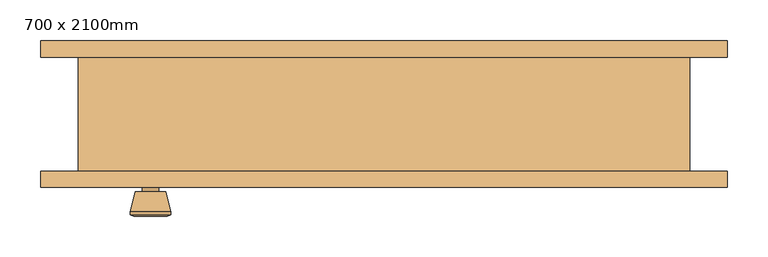
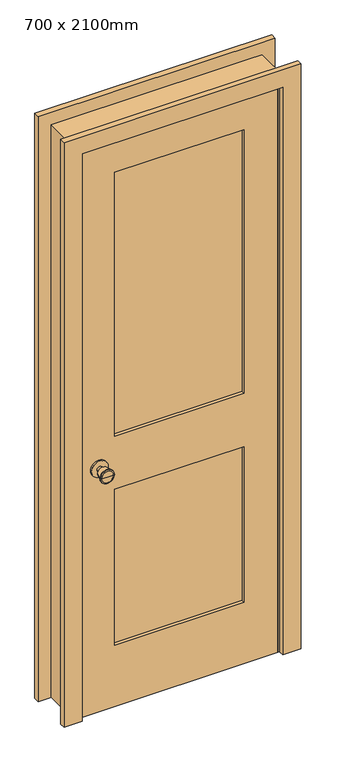
"""IFC4 building model written with IfcOpenShell, lengths in millimetres: door geometry, Porta-Interna-Única-2_Painel-Madeira : 700 x 2100mm."""

from ifc_helpers import new_model, si_unit, point, frame, frame_2d, origin, place, context, project, spatial, polyline, circle_curve, trimmed, segment, composite_curve, outline, extrude, faceted_brep, source, transform, mapped, element, save
from ifc_brep_helpers import plane_surface, cylinder_surface, revolved_surface, advanced_brep


def door_700_x_2100mm_1c1a1ff1(model_context):
    return source(origin(), model_context, "Body", "SolidModel", [
        advanced_brep(
        [(-286.5, -25.825, 914.4), (-296.5, -25.825, 914.4), (-276.5, -25.825, 914.4), (-266.0241324, 23.175, 914.4), (-306.9758676, 23.175, 914.4), (-286.5, 23.175, 914.4), (-261.5, 21.3471319, 914.4), (-311.5, 21.3471319, 914.4), (-261.5, 17.8834537, 914.4), (-311.5, 17.8834537, 914.4), (-267.863764, -6.825, 914.4), (-305.136236, -6.825, 914.4), (-276.5, -6.825, 914.4), (-296.5, -6.825, 914.4)],
        [
            (0, 1),
            (1, 2, circle_curve(frame((-286.5, -25.825, 914.4), z_axis=(0.0, -1.0, 0.0), x_axis=(-1.0, 0.0, 0.0)), 10.0)),
            (2, 0),
            (2, 1, circle_curve(frame((-286.5, -25.825, 914.4), z_axis=(0.0, -1.0, 0.0), x_axis=(-1.0, 0.0, 0.0)), 10.0)),
            (3, 4, circle_curve(frame((-286.5, 23.175, 914.4), z_axis=(0.0, 1.0, 0.0), x_axis=(-1.0, 0.0, 0.0)), 20.4758676)),
            (4, 5),
            (5, 3),
            (4, 3, circle_curve(frame((-286.5, 23.175, 914.4), z_axis=(0.0, 1.0, 0.0), x_axis=(-1.0, 0.0, 0.0)), 20.4758676)),
            (6, 7, circle_curve(frame((-286.5, 21.3471319, 914.4), z_axis=(0.0, 1.0, 0.0), x_axis=(-1.0, 0.0, 0.0)), 25.0)),
            (7, 4),
            (3, 6),
            (7, 6, circle_curve(frame((-286.5, 21.3471319, 914.4), z_axis=(0.0, 1.0, 0.0), x_axis=(-1.0, 0.0, 0.0)), 25.0)),
            (8, 9, circle_curve(frame((-286.5, 17.8834537, 914.4), z_axis=(0.0, 1.0, 0.0), x_axis=(-1.0, 0.0, 0.0)), 25.0)),
            (9, 7),
            (6, 8),
            (9, 8, circle_curve(frame((-286.5, 17.8834537, 914.4), z_axis=(0.0, 1.0, 0.0), x_axis=(-1.0, 0.0, 0.0)), 25.0)),
            (10, 11, circle_curve(frame((-286.5, -6.825, 914.4), z_axis=(0.0, 1.0, 0.0), x_axis=(-1.0, 0.0, 0.0)), 18.636236)),
            (11, 9),
            (8, 10),
            (11, 10, circle_curve(frame((-286.5, -6.825, 914.4), z_axis=(0.0, 1.0, 0.0), x_axis=(-1.0, 0.0, 0.0)), 18.636236)),
            (12, 13, circle_curve(frame((-286.5, -6.825, 914.4), z_axis=(0.0, 1.0, 0.0), x_axis=(-1.0, 0.0, 0.0)), 10.0)),
            (13, 11),
            (10, 12),
            (13, 12, circle_curve(frame((-286.5, -6.825, 914.4), z_axis=(0.0, 1.0, 0.0), x_axis=(-1.0, 0.0, 0.0)), 10.0)),
            (1, 13),
            (12, 2),
        ],
        [
            plane_surface(frame((-286.5, -25.825, 914.4), z_axis=(0.0, -1.0, 0.0), x_axis=(-1.0, 0.0, 0.0))),
            plane_surface(frame((-286.5, 23.175, 914.4), z_axis=(0.0, 1.0, 0.0), x_axis=(-1.0, 0.0, 0.0))),
            revolved_surface(polyline([(-306.9758676, 23.175, 914.4), (-311.5, 21.3471319, 914.4)]), (-286.5, -25.825, 914.4), (0.0, -1.0, 0.0)),
            cylinder_surface(frame((-286.5, -25.825, 914.4), z_axis=(0.0, -1.0, 0.0), x_axis=(-1.0, 0.0, 0.0)), 25.0),
            revolved_surface(polyline([(-311.5, 17.8834537, 914.4), (-305.136236, -6.825, 914.4)]), (-286.5, -25.825, 914.4), (0.0, -1.0, 0.0)),
            plane_surface(frame((-286.5, -6.825, 914.4), z_axis=(0.0, -1.0, 0.0), x_axis=(-1.0, 0.0, 0.0))),
            cylinder_surface(frame((-286.5, -25.825, 914.4), z_axis=(0.0, -1.0, 0.0), x_axis=(-1.0, 0.0, 0.0)), 10.0),
        ],
        [
            (0, [[1, 2, 3]]),
            (0, [[-3, 4, -1]]),
            (1, [[5, 6, 7]]),
            (1, [[8, -7, -6]]),
            (2, [[9, 10, -5, 11]]),
            (2, [[12, -11, -8, -10]]),
            (3, [[13, 14, -9, 15]]),
            (3, [[16, -15, -12, -14]]),
            (4, [[17, 18, -13, 19]]),
            (4, [[20, -19, -16, -18]]),
            (5, [[21, 22, -17, 23]]),
            (5, [[24, -23, -20, -22]]),
            (6, [[-2, 25, -21, 26]]),
            (6, [[-4, -26, -24, -25]]),
        ],
    ),
        extrude(outline(composite_curve([segment(trimmed(circle_curve(frame_2d((914.4, -286.5)), 30.0), [point((914.4, -316.5))], [point((914.4, -256.5))], False, "CARTESIAN"), True, "CONTINUOUS"), segment(trimmed(circle_curve(frame_2d((914.4, -286.5)), 30.0), [point((914.4, -256.5))], [point((914.4, -316.5))], False, "CARTESIAN"), True, "CONTINUOUS")], self_intersect=False)), frame((0.0, -31.825, 0.0), z_axis=(0.0, 1.0, 0.0), x_axis=(0.0, 0.0, 1.0)), (0.0, 0.0, 1.0), 6.0),
        advanced_brep(
        [(-286.5, -72.825, 914.4), (-276.5, -72.825, 914.4), (-296.5, -72.825, 914.4), (-266.0241324, -121.825, 914.4), (-286.5, -121.825, 914.4), (-306.9758676, -121.825, 914.4), (-261.5, -119.9971319, 914.4), (-311.5, -119.9971319, 914.4), (-261.5, -116.5334537, 914.4), (-311.5, -116.5334537, 914.4), (-267.863764, -91.825, 914.4), (-305.136236, -91.825, 914.4), (-276.5, -91.825, 914.4), (-296.5, -91.825, 914.4)],
        [
            (0, 1),
            (1, 2, circle_curve(frame((-286.5, -72.825, 914.4), z_axis=(0.0, 1.0, 0.0), x_axis=(-1.0, 0.0, 0.0)), 10.0)),
            (2, 0),
            (2, 1, circle_curve(frame((-286.5, -72.825, 914.4), z_axis=(0.0, 1.0, 0.0), x_axis=(-1.0, 0.0, 0.0)), 10.0)),
            (3, 4),
            (4, 5),
            (5, 3, circle_curve(frame((-286.5, -121.825, 914.4), z_axis=(0.0, -1.0, 0.0), x_axis=(-1.0, 0.0, 0.0)), 20.4758676)),
            (3, 5, circle_curve(frame((-286.5, -121.825, 914.4), z_axis=(0.0, -1.0, 0.0), x_axis=(-1.0, 0.0, 0.0)), 20.4758676)),
            (6, 3),
            (5, 7),
            (7, 6, circle_curve(frame((-286.5, -119.9971319, 914.4), z_axis=(0.0, -1.0, 0.0), x_axis=(-1.0, 0.0, 0.0)), 25.0)),
            (6, 7, circle_curve(frame((-286.5, -119.9971319, 914.4), z_axis=(0.0, -1.0, 0.0), x_axis=(-1.0, 0.0, 0.0)), 25.0)),
            (8, 6),
            (7, 9),
            (9, 8, circle_curve(frame((-286.5, -116.5334537, 914.4), z_axis=(0.0, -1.0, 0.0), x_axis=(-1.0, 0.0, 0.0)), 25.0)),
            (8, 9, circle_curve(frame((-286.5, -116.5334537, 914.4), z_axis=(0.0, -1.0, 0.0), x_axis=(-1.0, 0.0, 0.0)), 25.0)),
            (10, 8),
            (9, 11),
            (11, 10, circle_curve(frame((-286.5, -91.825, 914.4), z_axis=(0.0, -1.0, 0.0), x_axis=(-1.0, 0.0, 0.0)), 18.636236)),
            (10, 11, circle_curve(frame((-286.5, -91.825, 914.4), z_axis=(0.0, -1.0, 0.0), x_axis=(-1.0, 0.0, 0.0)), 18.636236)),
            (12, 10),
            (11, 13),
            (13, 12, circle_curve(frame((-286.5, -91.825, 914.4), z_axis=(0.0, -1.0, 0.0), x_axis=(-1.0, 0.0, 0.0)), 10.0)),
            (12, 13, circle_curve(frame((-286.5, -91.825, 914.4), z_axis=(0.0, -1.0, 0.0), x_axis=(-1.0, 0.0, 0.0)), 10.0)),
            (1, 12),
            (13, 2),
        ],
        [
            plane_surface(frame((-286.5, -72.825, 914.4), z_axis=(0.0, 1.0, 0.0), x_axis=(-1.0, 0.0, 0.0))),
            plane_surface(frame((-286.5, -121.825, 914.4), z_axis=(0.0, -1.0, 0.0), x_axis=(-1.0, 0.0, 0.0))),
            revolved_surface(polyline([(-306.9758676, -121.825, 914.4), (-311.5, -119.9971319, 914.4)]), (-286.5, -72.825, 914.4), (0.0, 1.0, 0.0)),
            cylinder_surface(frame((-286.5, -72.825, 914.4), z_axis=(0.0, 1.0, 0.0), x_axis=(-1.0, 0.0, 0.0)), 25.0),
            revolved_surface(polyline([(-311.5, -116.5334537, 914.4), (-305.136236, -91.825, 914.4)]), (-286.5, -72.825, 914.4), (0.0, 1.0, 0.0)),
            plane_surface(frame((-286.5, -91.825, 914.4), z_axis=(0.0, 1.0, 0.0), x_axis=(-1.0, 0.0, 0.0))),
            cylinder_surface(frame((-286.5, -72.825, 914.4), z_axis=(0.0, 1.0, 0.0), x_axis=(-1.0, 0.0, 0.0)), 10.0),
        ],
        [
            (0, [[1, 2, 3]]),
            (0, [[-3, 4, -1]]),
            (1, [[5, 6, 7]]),
            (1, [[-6, -5, 8]]),
            (2, [[9, -7, 10, 11]]),
            (2, [[-10, -8, -9, 12]]),
            (3, [[13, -11, 14, 15]]),
            (3, [[-14, -12, -13, 16]]),
            (4, [[17, -15, 18, 19]]),
            (4, [[-18, -16, -17, 20]]),
            (5, [[21, -19, 22, 23]]),
            (5, [[-22, -20, -21, 24]]),
            (6, [[25, -23, 26, -2]]),
            (6, [[-26, -24, -25, -4]]),
        ],
    ),
        extrude(outline(composite_curve([segment(trimmed(circle_curve(frame_2d((914.4, -286.5)), 30.0), [point((914.4, -316.5))], [point((914.4, -256.5))], False, "CARTESIAN"), True, "CONTINUOUS"), segment(trimmed(circle_curve(frame_2d((914.4, -286.5)), 30.0), [point((914.4, -256.5))], [point((914.4, -316.5))], False, "CARTESIAN"), True, "CONTINUOUS")], self_intersect=False)), frame((0.0, -72.825, 0.0), z_axis=(0.0, 1.0, 0.0), x_axis=(0.0, 0.0, 1.0)), (0.0, 0.0, 1.0), 6.0),
        extrude(outline(polyline([(230.0, -43.4916667), (230.0, -55.1583333), (-230.0, -55.1583333), (-230.0, -43.4916667), (230.0, -43.4916667)])), frame((0.0, 0.0, 1014.4), z_axis=(0.0, 0.0, 1.0), x_axis=(1.0, 0.0, 0.0)), (0.0, 0.0, 1.0), 990.6),
        extrude(outline(polyline([(230.0, -43.4916667), (230.0, -55.1583333), (-230.0, -55.1583333), (-230.0, -43.4916667), (230.0, -43.4916667)])), frame((0.0, 0.0, 230.0), z_axis=(0.0, 0.0, 1.0), x_axis=(1.0, 0.0, 0.0)), (0.0, 0.0, 1.0), 584.4),
        extrude(outline(polyline([(2125.0, -350.0), (0.0, -350.0), (0.0, 350.0), (2125.0, 350.0), (2125.0, -350.0)]), holes=[polyline([(2005.0, -230.0), (2005.0, 230.0), (1014.4, 230.0), (1014.4, -230.0), (2005.0, -230.0)]), polyline([(814.4, -230.0), (814.4, 230.0), (230.0, 230.0), (230.0, -230.0), (814.4, -230.0)])]), frame((0.0, -66.825, 0.0), z_axis=(0.0, 1.0, 0.0), x_axis=(0.0, 0.0, 1.0)), (0.0, 0.0, 1.0), 35.0),
        faceted_brep([(375.0, -66.825, 0.0), (350.0, -66.825, 0.0), (350.0, -31.825, 0.0), (337.3, -31.825, 0.0), (337.3, 3.1, 0.0), (350.0, 3.1, 0.0), (350.0, 73.175, 0.0), (375.0, 73.175, 0.0), (375.0, 73.175, 2150.0), (375.0, -66.825, 2150.0), (350.0, 73.175, 2125.0), (-350.0, 73.175, 2125.0), (-350.0, 73.175, 0.0), (-375.0, 73.175, 0.0), (-375.0, 73.175, 2150.0), (350.0, 3.1, 2125.0), (337.3, 3.1, 2112.3), (-337.3, 3.1, 2112.3), (-337.3, 3.1, 0.0), (-350.0, 3.1, 0.0), (-350.0, 3.1, 2125.0), (337.3, -31.825, 2112.3), (350.0, -31.825, 2125.0), (-350.0, -31.825, 2125.0), (-350.0, -31.825, 0.0), (-337.3, -31.825, 0.0), (-337.3, -31.825, 2112.3), (350.0, -66.825, 2125.0), (-375.0, -66.825, 2150.0), (-375.0, -66.825, 0.0), (-350.0, -66.825, 0.0), (-350.0, -66.825, 2125.0)], [[[0, 1, 2, 3, 4, 5, 6, 7]], [[7, 8, 9, 0]], [[6, 10, 11, 12, 13, 14, 8, 7]], [[5, 15, 10, 6]], [[4, 16, 17, 18, 19, 20, 15, 5]], [[3, 21, 16, 4]], [[2, 22, 23, 24, 25, 26, 21, 3]], [[1, 27, 22, 2]], [[0, 9, 28, 29, 30, 31, 27, 1]], [[8, 14, 28, 9]], [[15, 20, 11, 10]], [[21, 26, 17, 16]], [[27, 31, 23, 22]], [[29, 13, 12, 19, 18, 25, 24, 30]], [[14, 13, 29, 28]], [[20, 19, 12, 11]], [[26, 25, 18, 17]], [[31, 30, 24, 23]]]),
        extrude(outline(polyline([(0.0, 421.35), (2196.35, 421.35), (2196.35, -421.35), (0.0, -421.35), (0.0, -356.35), (2131.35, -356.35), (2131.35, 356.35), (0.0, 356.35), (0.0, 421.35)])), frame((0.0, 73.175, 0.0), z_axis=(0.0, 1.0, 0.0), x_axis=(0.0, 0.0, 1.0)), (0.0, 0.0, 1.0), 20.0),
        extrude(outline(polyline([(0.0, 421.35), (2196.35, 421.35), (2196.35, -421.35), (0.0, -421.35), (0.0, -356.35), (2131.35, -356.35), (2131.35, 356.35), (0.0, 356.35), (0.0, 421.35)])), frame((0.0, -86.825, 0.0), z_axis=(0.0, 1.0, 0.0), x_axis=(0.0, 0.0, 1.0)), (0.0, 0.0, 1.0), 20.0),
    ])


if __name__ == "__main__":
    model = new_model("IFC4")
    model_context = context("Model", 3, world=origin())
    ifc_project = project(units=[si_unit("LENGTHUNIT", "METRE", prefix="MILLI")], contexts=[model_context])
    site = spatial("IfcSite", under=ifc_project)
    building = spatial("IfcBuilding", under=site)
    placement = place(None, origin())
    door_700_x_2100mm_shape = door_700_x_2100mm_1c1a1ff1(model_context)
    element("IfcDoor", 1, ObjectType="Porta-Interna-Única-2_Painel-Madeira : 700 x 2100mm", at=placement, inside=building, context=model_context, shape_type="MappedRepresentation", body=[
        mapped(door_700_x_2100mm_shape, transform((0.0, 0.0, 0.0), x_axis=(1.0, 0.0, 0.0), y_axis=(0.0, 1.0, 0.0), z_axis=(0.0, 0.0, 1.0))),
    ])
    save(model, "model.ifc")

# Revit data of these elements
# Type "Porta-Interna-Única-2_Painel-Madeira : 700 x 2100mm"
#   Type Mark = "141"
#   Assembly Code = "C1020300"
#   Analytic Construction = "Madeira"
#   Corrimão superior = 0.120 m
#   Thickness = 0.035 m
#   Thermal Resistance (R) = 0.455703 (m²·K)/W
#   Ângulo de abertura [instance default] = 90.00°
#   Estilos = 0.120 m
#   Rough Width = 0.750 m
#   Rough Height = 2.150 m
#   Bloquear corrimão = 0.200 m
#   Height = 2.125 m
#   Width = 0.700 m
#   Heat Transfer Coefficient (U) = 2.19465 W/(m²·K)
#   Corrimão inferior = 0.230 m
#   Material da apara = Cerejeira
#   Material do painel = Cerejeira
#   Material da moldura = Cerejeira
#   Material da maçaneta = Alumín. 1
#   Visual Light Transmittance = 0
#   Solar Heat Gain Coefficient = 0
#   Wall Closure = (empty or 0)
#   Function = (empty or 0)
# Element 1 (IfcDoor, "Porta-Interna-Única-2_Painel-Madeira : 700 x 2100mm")
#   Materials on its faces: "Cerejeira", "Alumín. 1"
# Materials
#   "Cerejeira": class "Madeira", colour RGB 226 177 128, transparency 0, Description = "Prunus Serotina", Cost = 0
#   "Alumín. 1": class "Metal", colour RGB 247 247 247, transparency 0, Description = "Alumín. 6061", Cost = 0
